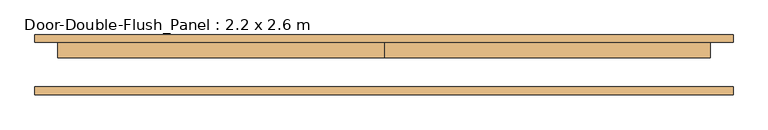
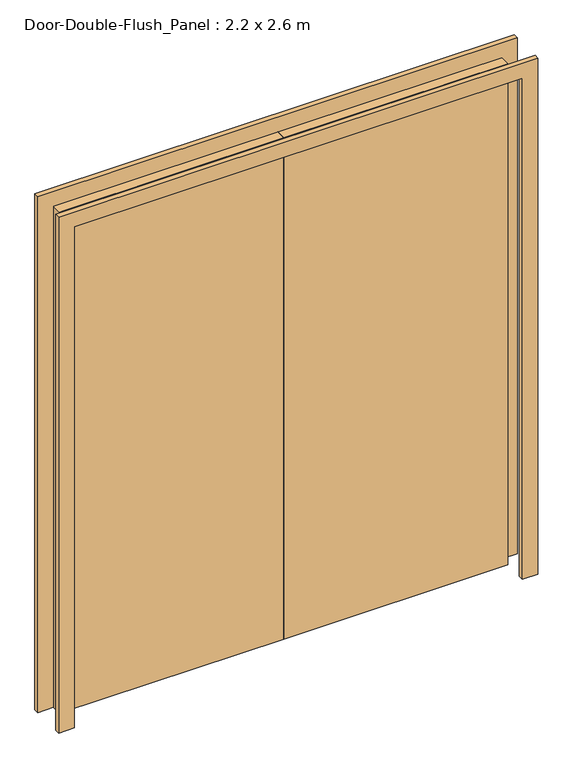
"""IFC4 building model written with IfcOpenShell, lengths in millimetres: door geometry, Door-Double-Flush_Panel : 2.2 x 2.6 m."""

from ifc_helpers import new_model, si_unit, frame, origin, origin_with_axes, place, context, project, spatial, polyline, outline, extrude, source, transform, mapped, element, save


def door_double_flush_panel_2_2_x_2_6_m_98fec84c(model_context):
    return source(origin(), model_context, "Body", "SweptSolid", [
        extrude(outline(polyline([(2600.0, -1100.0), (2600.0, 1100.0), (0.0, 1100.0), (0.0, 1176.2), (2676.2, 1176.2), (2676.2, -1176.2), (0.0, -1176.2), (0.0, -1100.0), (2600.0, -1100.0)])), frame((0.0, 75.0, 0.0), z_axis=(0.0, 1.0, 0.0), x_axis=(0.0, 0.0, 1.0)), (0.0, 0.0, 1.0), 25.4),
        extrude(outline(polyline([(2600.0, -1100.0), (2600.0, 1100.0), (0.0, 1100.0), (0.0, 1176.2), (2676.2, 1176.2), (2676.2, -1176.2), (0.0, -1176.2), (0.0, -1100.0), (2600.0, -1100.0)])), frame((0.0, -100.4, 0.0), z_axis=(0.0, 1.0, 0.0), x_axis=(0.0, 0.0, 1.0)), (0.0, 0.0, 1.0), 25.4),
        extrude(outline(polyline([(-1100.0, 75.0), (0.0, 75.0), (0.0, 24.2), (-1100.0, 24.2), (-1100.0, 75.0)])), origin_with_axes(), (0.0, 0.0, 1.0), 2600.0),
        extrude(outline(polyline([(0.0, 75.0), (1100.0, 75.0), (1100.0, 24.2), (0.0, 24.2), (0.0, 75.0)])), origin_with_axes(), (0.0, 0.0, 1.0), 2600.0),
    ])


if __name__ == "__main__":
    model = new_model("IFC4")
    model_context = context("Model", 3, world=origin())
    ifc_project = project(units=[si_unit("LENGTHUNIT", "METRE", prefix="MILLI")], contexts=[model_context])
    site = spatial("IfcSite", under=ifc_project)
    building = spatial("IfcBuilding", under=site)
    placement = place(None, origin())
    door_double_flush_panel_2_2_x_2_6_m_shape = door_double_flush_panel_2_2_x_2_6_m_98fec84c(model_context)
    element("IfcDoor", 1, ObjectType="Door-Double-Flush_Panel : 2.2 x 2.6 m", at=placement, inside=building, context=model_context, shape_type="MappedRepresentation", body=[
        mapped(door_double_flush_panel_2_2_x_2_6_m_shape, transform((0.0, 0.0, 0.0), x_axis=(1.0, 0.0, 0.0), y_axis=(0.0, 1.0, 0.0), z_axis=(0.0, 0.0, 1.0))),
    ])
    save(model, "model.ifc")

# Revit data of these elements
# Type "Door-Double-Flush_Panel : 2.2 x 2.6 m"
#   Type Mark = "49"
#   Construction Type Id = "DOOR"
#   Analytic Construction = "Wooden"
#   Thickness = 0.0508 m
#   Thermal Resistance (R) = 0.455703 (m²·K)/W
#   Swing Angle [instance default] = 90.00°
#   Panel Width = 1.1 m
#   Heat Transfer Coefficient (U) = 2.19465 W/(m²·K)
#   Height = 2.6 m
#   Trim Projection Ext = 0.0254 m
#   Trim Projection Int = 0.0254 m
#   Trim Width = 0.0762 m
#   Width = 2.2 m
#   Define Thermal Properties by = 1
#   Panel Material = Wood - Birch - Solid Stained Light Low Gloss
#   Trim Material = Paint - Sienna
#   Visual Light Transmittance = 0
#   Solar Heat Gain Coefficient = 0
#   Function = (empty or 0)
#   Wall Closure = (empty or 0)
# Element 1 (IfcDoor, "Door-Double-Flush_Panel : 2.2 x 2.6 m")
#   Materials on its faces: "Paint - Sienna", "Wood - Birch - Solid Stained Light Low Gloss"
# Materials
#   "Wood - Birch - Solid Stained Light Low Gloss": class "Wood", colour RGB 210 159 95, transparency 0, Cost = 0
#   "Paint - Sienna": class "Miscellaneous", colour RGB 118 70 51, transparency 0, Cost = 0
